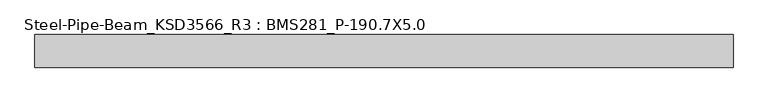
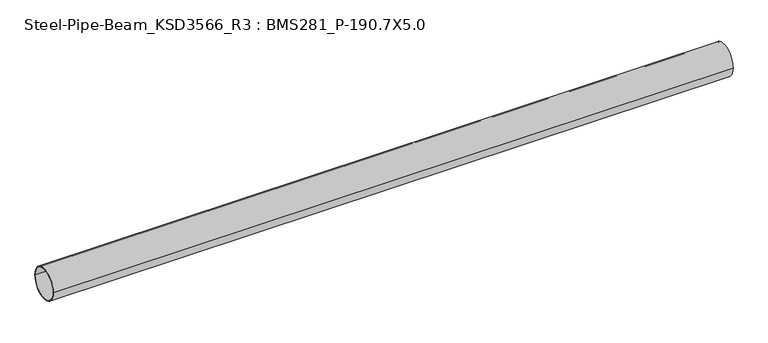
"""IFC4 building model written with IfcOpenShell, lengths in millimetres: member geometry, Steel-Pipe-Beam_KSD3566_R3 : BMS281_P-190.7X5.0."""

from ifc_helpers import new_model, si_unit, point, frame, origin, origin_2d, place, context, project, spatial, circle_curve, trimmed, segment, composite_curve, outline, extrude, source, transform, mapped, element, save


def steel_pipe_beam_ksd3566_r3_bms281_p_190_7x5_0_c2f906ac(model_context):
    return source(origin(), model_context, "Body", "SweptSolid", [
        extrude(outline(composite_curve([segment(trimmed(circle_curve(origin_2d(), 95.35), [point((-95.35, 0.0))], [point((95.35, 0.0))], False, "CARTESIAN"), True, "CONTINUOUS"), segment(trimmed(circle_curve(origin_2d(), 95.35), [point((95.35, 0.0))], [point((-95.35, 0.0))], False, "CARTESIAN"), True, "CONTINUOUS")], self_intersect=False), holes=[composite_curve([segment(trimmed(circle_curve(origin_2d(), 90.35), [point((90.35, 0.0))], [point((-90.35, 0.0))], True, "CARTESIAN"), True, "CONTINUOUS"), segment(trimmed(circle_curve(origin_2d(), 90.35), [point((-90.35, 0.0))], [point((90.35, 0.0))], True, "CARTESIAN"), True, "CONTINUOUS")], self_intersect=False)]), frame((-2031.1166586, 0.0, 0.0), z_axis=(1.0, 0.0, 0.0), x_axis=(0.0, 1.0, 0.0)), (0.0, 0.0, 1.0), 4077.9053115),
    ])


if __name__ == "__main__":
    model = new_model("IFC4")
    model_context = context("Model", 3, world=origin())
    ifc_project = project(units=[si_unit("LENGTHUNIT", "METRE", prefix="MILLI")], contexts=[model_context])
    site = spatial("IfcSite", under=ifc_project)
    building = spatial("IfcBuilding", under=site)
    placement = place(None, origin())
    steel_pipe_beam_ksd3566_r3_bms281_p_190_7x5_0_shape = steel_pipe_beam_ksd3566_r3_bms281_p_190_7x5_0_c2f906ac(model_context)
    element("IfcMember", 1, ObjectType="Steel-Pipe-Beam_KSD3566_R3 : BMS281_P-190.7X5.0", at=placement, inside=building, context=model_context, shape_type="MappedRepresentation", body=[
        mapped(steel_pipe_beam_ksd3566_r3_bms281_p_190_7x5_0_shape, transform((0.0, 0.0, 0.0), x_axis=(1.0, 0.0, 0.0), y_axis=(0.0, 1.0, 0.0), z_axis=(0.0, 0.0, 1.0))),
    ])
    save(model, "model.ifc")

# Revit data of these elements
# Type "Steel-Pipe-Beam_KSD3566_R3 : BMS281_P-190.7X5.0"
#   Keynote = "P-190.7X5.0"
#   SteelWeight = "Light"
#   t = 0.0050 m
#   Surface Area = 0.599102 m²/m
#   Section Area = 29.1697 cm²
#   Mass per Unit Length = 22.8982 kg/m
#   Length [instance default] = 1.5000 m
#   D = 0.1907 m
#   hec_material4 [instance default] = none
#   hec_material3 [instance default] = none
#   hec_material2 [instance default] = none
#   hec_material1 [instance default] = none
#   Structural Material [instance default] = Steel, 45-345
#   Assembly Code = ""
# Element 1 (IfcMember, "Steel-Pipe-Beam_KSD3566_R3 : BMS281_P-190.7X5.0")
#   Structural Material = none
# Materials
#   "Steel, 45-345": class "Metal", colour RGB 189 187 185, transparency 0, Description = "Steel 345 MPa", Cost = 0
